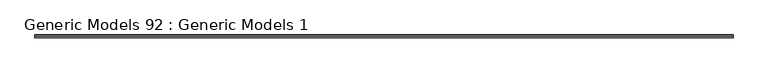
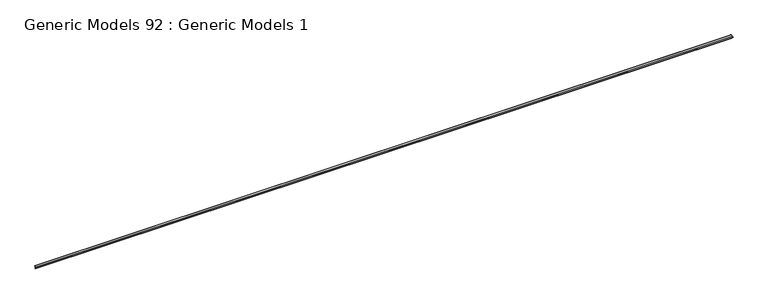
"""IFC4 building model written with IfcOpenShell, lengths in millimetres: proxy geometry, Generic Models 92 : Generic Models 1."""

from ifc_helpers import new_model, si_unit, point, frame, frame_2d, origin, place, context, project, spatial, polyline, circle_curve, trimmed, segment, composite_curve, outline, extrude, source, transform, mapped, element, save


def generic_models_92_generic_models_1_77b13597(model_context):
    return source(origin(), model_context, "Body", "SweptSolid", [
        extrude(outline(composite_curve([segment(trimmed(circle_curve(frame_2d((51514.4033415, 127165.3167873)), 1.4342127), [point((51513.7481865, 127166.5926156))], [point((51515.6791698, 127164.6616323))], False, "CARTESIAN"), True, "CONTINUOUS"), segment(polyline([(51515.6791698, 127164.6616323), (51496.1525542, 127126.6361176), (51496.1525542, 127088.5361176), (51494.8825542, 127088.5361176), (51494.8825542, 127126.9431414), (51514.7827938, 127165.6962396), (51476.0296956, 127145.796), (51437.6226718, 127145.796), (51437.6226718, 127147.066), (51475.7226718, 127147.066), (51513.7481865, 127166.5926156)]), True, "CONTINUOUS")], self_intersect=False)), frame((-20998.9733045, 0.0, 0.0), z_axis=(1.0, 0.0, 0.0), x_axis=(0.0, 1.0, 0.0)), (0.0, 0.0, 1.0), 19050.0),
    ])


if __name__ == "__main__":
    model = new_model("IFC4")
    model_context = context("Model", 3, world=origin())
    ifc_project = project(units=[si_unit("LENGTHUNIT", "METRE", prefix="MILLI")], contexts=[model_context])
    site = spatial("IfcSite", under=ifc_project)
    building = spatial("IfcBuilding", under=site)
    placement = place(None, origin())
    generic_models_92_generic_models_1_shape = generic_models_92_generic_models_1_77b13597(model_context)
    element("IfcBuildingElementProxy", 1, Name="Generic Models 92 : Generic Models 1", ObjectType="Generic Models 92 : Generic Models 1", at=placement, inside=building, context=model_context, shape_type="MappedRepresentation", body=[
        mapped(generic_models_92_generic_models_1_shape, transform((0.0, 0.0, 0.0), x_axis=(1.0, 0.0, 0.0), y_axis=(0.0, 1.0, 0.0), z_axis=(0.0, 0.0, 1.0))),
    ])
    save(model, "model.ifc")

# Revit data of these elements
# Element 1 (IfcBuildingElementProxy, "Generic Models 92 : Generic Models 1")
#   Materials on its faces: "_CONTINIOUS 16 GA. COPPER CORNER BEAD"
# Materials
#   "_CONTINIOUS 16 GA. COPPER CORNER BEAD": class "Generic", colour RGB 253 192 103, transparency 0, Cost = 0
